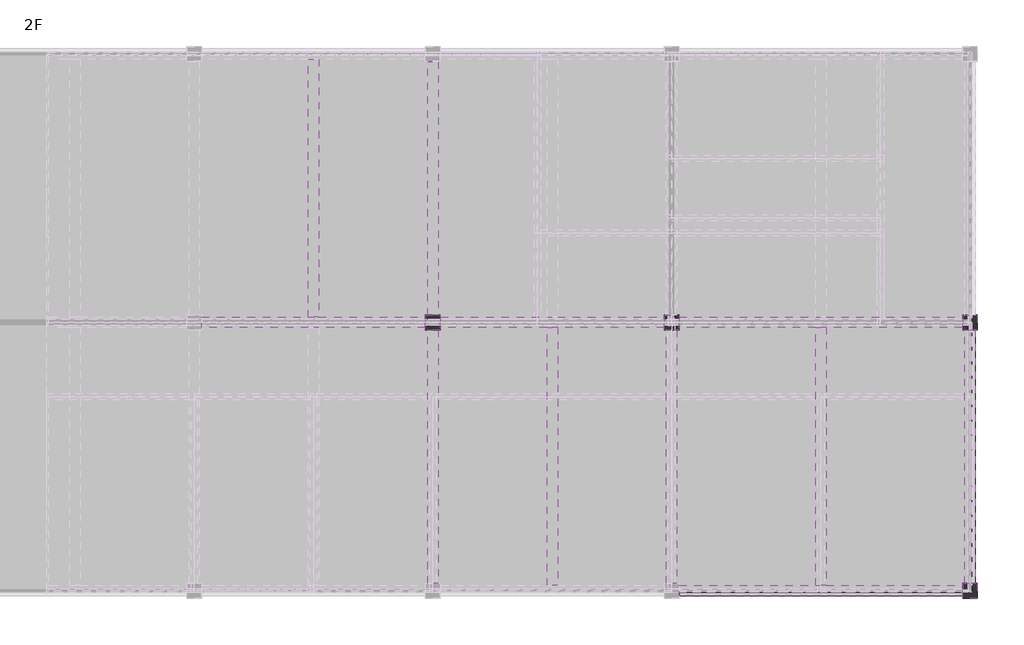
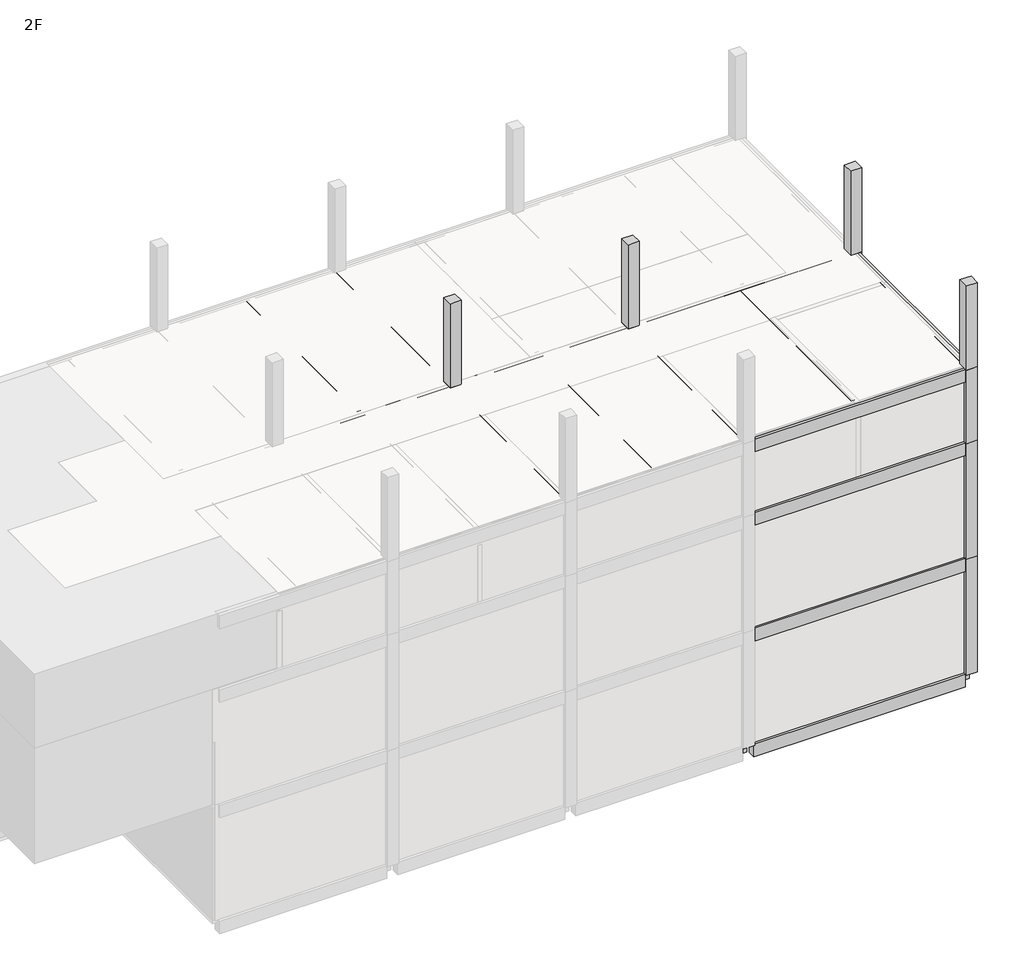
# One storey, part 6 of 7: 42 beams, 16 columns.
"""IFC4 building model written with IfcOpenShell, lengths in millimetres."""

from ifc_helpers import new_model, si_unit, frame, origin, place, context, project, spatial, polyline, outline, extrude, faceted_brep, element, save

model = new_model("IFC4")

# Units and contexts
model_context = context("Model", 3, world=origin())
ifc_project = project(units=[si_unit("LENGTHUNIT", "METRE", prefix="MILLI")], contexts=[model_context])

# Site, building, storey
site = spatial("IfcSite", under=ifc_project)
building = spatial("IfcBuilding", under=site)
storey = spatial("IfcBuildingStorey", under=building, Name="2F", Elevation=3500.0)

# Beams
placement = place(None, origin())
element("IfcBeam", 1, ObjectType="Concrete-Rectangular-Beam : BM111_400x500_RG1", at=placement, inside=storey, context=model_context, shape_type="SweptSolid", body=[
    extrude(outline(polyline([(65634.6521483, 173098.8614395), (65284.6521483, 173098.8614395), (65284.6521483, 181748.8614395), (65634.6521483, 181748.8614395), (65634.6521483, 173098.8614395)])), frame((0.0, 0.0, 2900.0), z_axis=(0.0, 0.0, 1.0), x_axis=(1.0, 0.0, 0.0)), (0.0, 0.0, 1.0), 600.0),
])
element("IfcBeam", 2, ObjectType="Concrete-Rectangular-Beam : BM111_400x500_RG1", at=placement, inside=storey, context=model_context, shape_type="SweptSolid", body=[
    extrude(outline(polyline([(73284.6521483, 172748.8614395), (73634.6521483, 172748.8614395), (73634.6521483, 164098.8614395), (73284.6521483, 164098.8614395), (73284.6521483, 172748.8614395)])), frame((0.0, 0.0, 2900.0), z_axis=(0.0, 0.0, 1.0), x_axis=(1.0, 0.0, 0.0)), (0.0, 0.0, 1.0), 600.0),
])
element("IfcBeam", 3, ObjectType="Concrete-Rectangular-Beam : BM111_400x500_RG1", at=placement, inside=storey, context=model_context, shape_type="SweptSolid", body=[
    extrude(outline(polyline([(82284.6521483, 172748.8614395), (82634.6521483, 172748.8614395), (82634.6521483, 164098.8614395), (82284.6521483, 164098.8614395), (82284.6521483, 172748.8614395)])), frame((0.0, 0.0, 2900.0), z_axis=(0.0, 0.0, 1.0), x_axis=(1.0, 0.0, 0.0)), (0.0, 0.0, 1.0), 600.0),
])
element("IfcBeam", 4, ObjectType="Concrete-Rectangular-Beam : BM111_400x500_RG1", at=placement, inside=storey, context=model_context, shape_type="SweptSolid", body=[
    extrude(outline(polyline([(65634.6521483, 173098.8614395), (65284.6521483, 173098.8614395), (65284.6521483, 181748.8614395), (65634.6521483, 181748.8614395), (65634.6521483, 173098.8614395)])), frame((0.0, 0.0, 8400.0), z_axis=(0.0, 0.0, 1.0), x_axis=(1.0, 0.0, 0.0)), (0.0, 0.0, 1.0), 600.0),
])
element("IfcBeam", 5, ObjectType="Concrete-Rectangular-Beam : BM111_400x500_RG1", at=placement, inside=storey, context=model_context, shape_type="SweptSolid", body=[
    extrude(outline(polyline([(73284.6521483, 172748.8614395), (73634.6521483, 172748.8614395), (73634.6521483, 164098.8614395), (73284.6521483, 164098.8614395), (73284.6521483, 172748.8614395)])), frame((0.0, 0.0, 8400.0), z_axis=(0.0, 0.0, 1.0), x_axis=(1.0, 0.0, 0.0)), (0.0, 0.0, 1.0), 600.0),
])
element("IfcBeam", 6, ObjectType="Concrete-Rectangular-Beam : BM111_400x500_RG1", at=placement, inside=storey, context=model_context, shape_type="SweptSolid", body=[
    extrude(outline(polyline([(82284.6521483, 172748.8614395), (82634.6521483, 172748.8614395), (82634.6521483, 164098.8614395), (82284.6521483, 164098.8614395), (82284.6521483, 172748.8614395)])), frame((0.0, 0.0, 8400.0), z_axis=(0.0, 0.0, 1.0), x_axis=(1.0, 0.0, 0.0)), (0.0, 0.0, 1.0), 600.0),
])
element("IfcBeam", 7, ObjectType="Concrete-Rectangular-Beam : BM111_400x500_RG1", at=placement, inside=storey, context=model_context, shape_type="SweptSolid", body=[
    extrude(outline(polyline([(65634.6521483, 173098.8614395), (65284.6521483, 173098.8614395), (65284.6521483, 181748.8614395), (65634.6521483, 181748.8614395), (65634.6521483, 173098.8614395)])), frame((0.0, 0.0, 13900.0), z_axis=(0.0, 0.0, 1.0), x_axis=(1.0, 0.0, 0.0)), (0.0, 0.0, 1.0), 600.0),
])
element("IfcBeam", 8, ObjectType="Concrete-Rectangular-Beam : BM111_400x500_RG1", at=placement, inside=storey, context=model_context, shape_type="SweptSolid", body=[
    extrude(outline(polyline([(73284.6521483, 172748.8614395), (73634.6521483, 172748.8614395), (73634.6521483, 164098.8614395), (73284.6521483, 164098.8614395), (73284.6521483, 172748.8614395)])), frame((0.0, 0.0, 13900.0), z_axis=(0.0, 0.0, 1.0), x_axis=(1.0, 0.0, 0.0)), (0.0, 0.0, 1.0), 600.0),
])
element("IfcBeam", 9, ObjectType="Concrete-Rectangular-Beam : BM111_400x500_RG1", at=placement, inside=storey, context=model_context, shape_type="SweptSolid", body=[
    extrude(outline(polyline([(82284.6521483, 172748.8614395), (82634.6521483, 172748.8614395), (82634.6521483, 164098.8614395), (82284.6521483, 164098.8614395), (82284.6521483, 172748.8614395)])), frame((0.0, 0.0, 13900.0), z_axis=(0.0, 0.0, 1.0), x_axis=(1.0, 0.0, 0.0)), (0.0, 0.0, 1.0), 600.0),
])
element("IfcBeam", 10, ObjectType="Concrete-Rectangular-Beam : BM111_400x500_RG1", at=placement, inside=storey, context=model_context, shape_type="SweptSolid", body=[
    extrude(outline(polyline([(65634.6521483, 173098.8614395), (65284.6521483, 173098.8614395), (65284.6521483, 181748.8614395), (65634.6521483, 181748.8614395), (65634.6521483, 173098.8614395)])), frame((0.0, 0.0, 17400.0), z_axis=(0.0, 0.0, 1.0), x_axis=(1.0, 0.0, 0.0)), (0.0, 0.0, 1.0), 600.0),
])
element("IfcBeam", 11, ObjectType="Concrete-Rectangular-Beam : BM111_400x500_RG1", at=placement, inside=storey, context=model_context, shape_type="SweptSolid", body=[
    extrude(outline(polyline([(73284.6521483, 172748.8614395), (73634.6521483, 172748.8614395), (73634.6521483, 164098.8614395), (73284.6521483, 164098.8614395), (73284.6521483, 172748.8614395)])), frame((0.0, 0.0, 17400.0), z_axis=(0.0, 0.0, 1.0), x_axis=(1.0, 0.0, 0.0)), (0.0, 0.0, 1.0), 600.0),
])
element("IfcBeam", 12, ObjectType="Concrete-Rectangular-Beam : BM111_400x500_RG1", at=placement, inside=storey, context=model_context, shape_type="SweptSolid", body=[
    extrude(outline(polyline([(82284.6521483, 172748.8614395), (82634.6521483, 172748.8614395), (82634.6521483, 164098.8614395), (82284.6521483, 164098.8614395), (82284.6521483, 172748.8614395)])), frame((0.0, 0.0, 17400.0), z_axis=(0.0, 0.0, 1.0), x_axis=(1.0, 0.0, 0.0)), (0.0, 0.0, 1.0), 600.0),
])
element("IfcBeam", 13, ObjectType="Concrete-Rectangular-Beam : BM111_400x500_RG1", at=placement, inside=storey, context=model_context, shape_type="Brep", body=[
    faceted_brep([(61709.6521483, 173098.8614395, 3500.0), (61709.6521483, 172748.8614395, 3500.0), (65284.6521483, 172748.8614395, 3500.0), (65634.6521483, 172748.8614395, 3500.0), (69209.6521483, 172748.8614395, 3500.0), (69209.6521483, 173098.8614395, 3500.0), (65634.6521483, 173098.8614395, 3500.0), (65284.6521483, 173098.8614395, 3500.0), (61709.6521483, 172748.8614395, 2900.0), (65284.6521483, 172748.8614395, 2900.0), (65634.6521483, 172748.8614395, 2900.0), (69209.6521483, 172748.8614395, 2900.0), (61709.6521483, 173098.8614395, 2900.0), (65284.6521483, 173098.8614395, 2900.0), (65634.6521483, 173098.8614395, 2900.0), (69209.6521483, 173098.8614395, 2900.0)], [[[0, 1, 2, 3, 4, 5, 6, 7]], [[1, 8, 9, 10, 11, 4, 3, 2]], [[8, 12, 13, 14, 15, 11, 10, 9]], [[12, 0, 7, 6, 5, 15, 14, 13]], [[1, 0, 12, 8]], [[5, 4, 11, 15]]]),
])
element("IfcBeam", 14, ObjectType="Concrete-Rectangular-Beam : BM111_400x500_RG1", at=placement, inside=storey, context=model_context, shape_type="Brep", body=[
    faceted_brep([(69709.6521483, 173098.8614395, 3500.0), (69709.6521483, 172748.8614395, 3500.0), (73284.6521483, 172748.8614395, 3500.0), (73634.6521483, 172748.8614395, 3500.0), (77209.6521483, 172748.8614395, 3500.0), (77209.6521483, 173098.8614395, 3500.0), (73634.6521483, 173098.8614395, 3500.0), (73284.6521483, 173098.8614395, 3500.0), (69709.6521483, 172748.8614395, 2900.0), (73284.6521483, 172748.8614395, 2900.0), (73634.6521483, 172748.8614395, 2900.0), (77209.6521483, 172748.8614395, 2900.0), (69709.6521483, 173098.8614395, 2900.0), (73284.6521483, 173098.8614395, 2900.0), (73634.6521483, 173098.8614395, 2900.0), (77209.6521483, 173098.8614395, 2900.0)], [[[0, 1, 2, 3, 4, 5, 6, 7]], [[1, 8, 9, 10, 11, 4, 3, 2]], [[8, 12, 13, 14, 15, 11, 10, 9]], [[12, 0, 7, 6, 5, 15, 14, 13]], [[1, 0, 12, 8]], [[5, 4, 11, 15]]]),
])
element("IfcBeam", 15, ObjectType="Concrete-Rectangular-Beam : BM111_400x500_RG1", at=placement, inside=storey, context=model_context, shape_type="Brep", body=[
    faceted_brep([(77709.6521483, 173098.8614395, 3500.0), (77709.6521483, 172748.8614395, 3500.0), (82284.6521483, 172748.8614395, 3500.0), (82634.6521483, 172748.8614395, 3500.0), (87209.6521483, 172748.8614395, 3500.0), (87209.6521483, 173098.8614395, 3500.0), (82634.6521483, 173098.8614395, 3500.0), (82284.6521483, 173098.8614395, 3500.0), (77709.6521483, 172748.8614395, 2900.0), (82284.6521483, 172748.8614395, 2900.0), (82634.6521483, 172748.8614395, 2900.0), (87209.6521483, 172748.8614395, 2900.0), (77709.6521483, 173098.8614395, 2900.0), (82284.6521483, 173098.8614395, 2900.0), (82634.6521483, 173098.8614395, 2900.0), (87209.6521483, 173098.8614395, 2900.0)], [[[0, 1, 2, 3, 4, 5, 6, 7]], [[1, 8, 9, 10, 11, 4, 3, 2]], [[8, 12, 13, 14, 15, 11, 10, 9]], [[12, 0, 7, 6, 5, 15, 14, 13]], [[1, 0, 12, 8]], [[5, 4, 11, 15]]]),
])
element("IfcBeam", 16, ObjectType="Concrete-Rectangular-Beam : BM111_400x500_RG1", at=placement, inside=storey, context=model_context, shape_type="Brep", body=[
    faceted_brep([(77709.6521483, 164098.8614395, 3500.0), (77709.6521483, 163748.8614395, 3500.0), (87209.6521483, 163748.8614395, 3500.0), (87209.6521483, 164098.8614395, 3500.0), (82634.6521483, 164098.8614395, 3500.0), (82284.6521483, 164098.8614395, 3500.0), (77709.6521483, 163748.8614395, 2900.0), (87209.6521483, 163748.8614395, 2900.0), (77709.6521483, 164098.8614395, 2900.0), (82284.6521483, 164098.8614395, 2900.0), (82634.6521483, 164098.8614395, 2900.0), (87209.6521483, 164098.8614395, 2900.0)], [[[0, 1, 2, 3, 4, 5]], [[1, 6, 7, 2]], [[6, 8, 9, 10, 11, 7]], [[8, 0, 5, 4, 3, 11, 10, 9]], [[1, 0, 8, 6]], [[3, 2, 7, 11]]]),
])
element("IfcBeam", 17, ObjectType="Concrete-Rectangular-Beam : BM111_400x500_RG1", at=placement, inside=storey, context=model_context, shape_type="Brep", body=[
    faceted_brep([(61709.6521483, 173098.8614395, 9000.0), (61709.6521483, 172748.8614395, 9000.0), (65284.6521483, 172748.8614395, 9000.0), (65634.6521483, 172748.8614395, 9000.0), (69209.6521483, 172748.8614395, 9000.0), (69209.6521483, 173098.8614395, 9000.0), (65634.6521483, 173098.8614395, 9000.0), (65284.6521483, 173098.8614395, 9000.0), (61709.6521483, 172748.8614395, 8400.0), (65284.6521483, 172748.8614395, 8400.0), (65634.6521483, 172748.8614395, 8400.0), (69209.6521483, 172748.8614395, 8400.0), (61709.6521483, 173098.8614395, 8400.0), (65284.6521483, 173098.8614395, 8400.0), (65634.6521483, 173098.8614395, 8400.0), (69209.6521483, 173098.8614395, 8400.0)], [[[0, 1, 2, 3, 4, 5, 6, 7]], [[1, 8, 9, 10, 11, 4, 3, 2]], [[8, 12, 13, 14, 15, 11, 10, 9]], [[12, 0, 7, 6, 5, 15, 14, 13]], [[1, 0, 12, 8]], [[5, 4, 11, 15]]]),
])
element("IfcBeam", 18, ObjectType="Concrete-Rectangular-Beam : BM111_400x500_RG1", at=placement, inside=storey, context=model_context, shape_type="Brep", body=[
    faceted_brep([(69709.6521483, 173098.8614395, 9000.0), (69709.6521483, 172748.8614395, 9000.0), (73284.6521483, 172748.8614395, 9000.0), (73634.6521483, 172748.8614395, 9000.0), (77209.6521483, 172748.8614395, 9000.0), (77209.6521483, 173098.8614395, 9000.0), (73634.6521483, 173098.8614395, 9000.0), (73284.6521483, 173098.8614395, 9000.0), (69709.6521483, 172748.8614395, 8400.0), (73284.6521483, 172748.8614395, 8400.0), (73634.6521483, 172748.8614395, 8400.0), (77209.6521483, 172748.8614395, 8400.0), (69709.6521483, 173098.8614395, 8400.0), (73284.6521483, 173098.8614395, 8400.0), (73634.6521483, 173098.8614395, 8400.0), (77209.6521483, 173098.8614395, 8400.0)], [[[0, 1, 2, 3, 4, 5, 6, 7]], [[1, 8, 9, 10, 11, 4, 3, 2]], [[8, 12, 13, 14, 15, 11, 10, 9]], [[12, 0, 7, 6, 5, 15, 14, 13]], [[1, 0, 12, 8]], [[5, 4, 11, 15]]]),
])
element("IfcBeam", 19, ObjectType="Concrete-Rectangular-Beam : BM111_400x500_RG1", at=placement, inside=storey, context=model_context, shape_type="Brep", body=[
    faceted_brep([(77709.6521483, 173098.8614395, 9000.0), (77709.6521483, 172748.8614395, 9000.0), (82284.6521483, 172748.8614395, 9000.0), (82634.6521483, 172748.8614395, 9000.0), (87209.6521483, 172748.8614395, 9000.0), (87209.6521483, 173098.8614395, 9000.0), (82634.6521483, 173098.8614395, 9000.0), (82284.6521483, 173098.8614395, 9000.0), (77709.6521483, 172748.8614395, 8400.0), (82284.6521483, 172748.8614395, 8400.0), (82634.6521483, 172748.8614395, 8400.0), (87209.6521483, 172748.8614395, 8400.0), (77709.6521483, 173098.8614395, 8400.0), (82284.6521483, 173098.8614395, 8400.0), (82634.6521483, 173098.8614395, 8400.0), (87209.6521483, 173098.8614395, 8400.0)], [[[0, 1, 2, 3, 4, 5, 6, 7]], [[1, 8, 9, 10, 11, 4, 3, 2]], [[8, 12, 13, 14, 15, 11, 10, 9]], [[12, 0, 7, 6, 5, 15, 14, 13]], [[1, 0, 12, 8]], [[5, 4, 11, 15]]]),
])
element("IfcBeam", 20, ObjectType="Concrete-Rectangular-Beam : BM111_400x500_RG1", at=placement, inside=storey, context=model_context, shape_type="Brep", body=[
    faceted_brep([(77709.6521483, 164098.8614395, 9000.0), (77709.6521483, 163748.8614395, 9000.0), (87209.6521483, 163748.8614395, 9000.0), (87209.6521483, 164098.8614395, 9000.0), (82634.6521483, 164098.8614395, 9000.0), (82284.6521483, 164098.8614395, 9000.0), (77709.6521483, 163748.8614395, 8400.0), (87209.6521483, 163748.8614395, 8400.0), (77709.6521483, 164098.8614395, 8400.0), (82284.6521483, 164098.8614395, 8400.0), (82634.6521483, 164098.8614395, 8400.0), (87209.6521483, 164098.8614395, 8400.0)], [[[0, 1, 2, 3, 4, 5]], [[1, 6, 7, 2]], [[6, 8, 9, 10, 11, 7]], [[8, 0, 5, 4, 3, 11, 10, 9]], [[1, 0, 8, 6]], [[3, 2, 7, 11]]]),
])
element("IfcBeam", 21, ObjectType="Concrete-Rectangular-Beam : BM111_400x500_RG1", at=placement, inside=storey, context=model_context, shape_type="Brep", body=[
    faceted_brep([(61709.6521483, 173098.8614395, 14500.0), (61709.6521483, 172748.8614395, 14500.0), (65284.6521483, 172748.8614395, 14500.0), (65634.6521483, 172748.8614395, 14500.0), (69209.6521483, 172748.8614395, 14500.0), (69209.6521483, 173098.8614395, 14500.0), (65634.6521483, 173098.8614395, 14500.0), (65284.6521483, 173098.8614395, 14500.0), (61709.6521483, 172748.8614395, 13900.0), (65284.6521483, 172748.8614395, 13900.0), (65634.6521483, 172748.8614395, 13900.0), (69209.6521483, 172748.8614395, 13900.0), (61709.6521483, 173098.8614395, 13900.0), (65284.6521483, 173098.8614395, 13900.0), (65634.6521483, 173098.8614395, 13900.0), (69209.6521483, 173098.8614395, 13900.0)], [[[0, 1, 2, 3, 4, 5, 6, 7]], [[1, 8, 9, 10, 11, 4, 3, 2]], [[8, 12, 13, 14, 15, 11, 10, 9]], [[12, 0, 7, 6, 5, 15, 14, 13]], [[1, 0, 12, 8]], [[5, 4, 11, 15]]]),
])
element("IfcBeam", 22, ObjectType="Concrete-Rectangular-Beam : BM111_400x500_RG1", at=placement, inside=storey, context=model_context, shape_type="Brep", body=[
    faceted_brep([(69709.6521483, 173098.8614395, 14500.0), (69709.6521483, 172748.8614395, 14500.0), (73284.6521483, 172748.8614395, 14500.0), (73634.6521483, 172748.8614395, 14500.0), (77209.6521483, 172748.8614395, 14500.0), (77209.6521483, 173098.8614395, 14500.0), (73634.6521483, 173098.8614395, 14500.0), (73284.6521483, 173098.8614395, 14500.0), (69709.6521483, 172748.8614395, 13900.0), (73284.6521483, 172748.8614395, 13900.0), (73634.6521483, 172748.8614395, 13900.0), (77209.6521483, 172748.8614395, 13900.0), (69709.6521483, 173098.8614395, 13900.0), (73284.6521483, 173098.8614395, 13900.0), (73634.6521483, 173098.8614395, 13900.0), (77209.6521483, 173098.8614395, 13900.0)], [[[0, 1, 2, 3, 4, 5, 6, 7]], [[1, 8, 9, 10, 11, 4, 3, 2]], [[8, 12, 13, 14, 15, 11, 10, 9]], [[12, 0, 7, 6, 5, 15, 14, 13]], [[1, 0, 12, 8]], [[5, 4, 11, 15]]]),
])
element("IfcBeam", 23, ObjectType="Concrete-Rectangular-Beam : BM111_400x500_RG1", at=placement, inside=storey, context=model_context, shape_type="Brep", body=[
    faceted_brep([(77709.6521483, 173098.8614395, 14500.0), (77709.6521483, 172748.8614395, 14500.0), (82284.6521483, 172748.8614395, 14500.0), (82634.6521483, 172748.8614395, 14500.0), (87209.6521483, 172748.8614395, 14500.0), (87209.6521483, 173098.8614395, 14500.0), (82634.6521483, 173098.8614395, 14500.0), (82284.6521483, 173098.8614395, 14500.0), (77709.6521483, 172748.8614395, 13900.0), (82284.6521483, 172748.8614395, 13900.0), (82634.6521483, 172748.8614395, 13900.0), (87209.6521483, 172748.8614395, 13900.0), (77709.6521483, 173098.8614395, 13900.0), (82284.6521483, 173098.8614395, 13900.0), (82634.6521483, 173098.8614395, 13900.0), (87209.6521483, 173098.8614395, 13900.0)], [[[0, 1, 2, 3, 4, 5, 6, 7]], [[1, 8, 9, 10, 11, 4, 3, 2]], [[8, 12, 13, 14, 15, 11, 10, 9]], [[12, 0, 7, 6, 5, 15, 14, 13]], [[1, 0, 12, 8]], [[5, 4, 11, 15]]]),
])
element("IfcBeam", 24, ObjectType="Concrete-Rectangular-Beam : BM111_400x500_RG1", at=placement, inside=storey, context=model_context, shape_type="Brep", body=[
    faceted_brep([(77709.6521483, 164098.8614395, 14500.0), (77709.6521483, 163748.8614395, 14500.0), (87209.6521483, 163748.8614395, 14500.0), (87209.6521483, 164098.8614395, 14500.0), (82634.6521483, 164098.8614395, 14500.0), (82284.6521483, 164098.8614395, 14500.0), (77709.6521483, 163748.8614395, 13900.0), (87209.6521483, 163748.8614395, 13900.0), (77709.6521483, 164098.8614395, 13900.0), (82284.6521483, 164098.8614395, 13900.0), (82634.6521483, 164098.8614395, 13900.0), (87209.6521483, 164098.8614395, 13900.0)], [[[0, 1, 2, 3, 4, 5]], [[1, 6, 7, 2]], [[6, 8, 9, 10, 11, 7]], [[8, 0, 5, 4, 3, 11, 10, 9]], [[1, 0, 8, 6]], [[3, 2, 7, 11]]]),
])
element("IfcBeam", 25, ObjectType="Concrete-Rectangular-Beam : BM111_400x500_RG1", at=placement, inside=storey, context=model_context, shape_type="Brep", body=[
    faceted_brep([(61709.6521483, 173098.8614395, 18000.0), (61709.6521483, 172748.8614395, 18000.0), (65284.6521483, 172748.8614395, 18000.0), (65634.6521483, 172748.8614395, 18000.0), (69209.6521483, 172748.8614395, 18000.0), (69209.6521483, 173098.8614395, 18000.0), (65634.6521483, 173098.8614395, 18000.0), (65284.6521483, 173098.8614395, 18000.0), (61709.6521483, 172748.8614395, 17400.0), (65284.6521483, 172748.8614395, 17400.0), (65634.6521483, 172748.8614395, 17400.0), (69209.6521483, 172748.8614395, 17400.0), (61709.6521483, 173098.8614395, 17400.0), (65284.6521483, 173098.8614395, 17400.0), (65634.6521483, 173098.8614395, 17400.0), (69209.6521483, 173098.8614395, 17400.0)], [[[0, 1, 2, 3, 4, 5, 6, 7]], [[1, 8, 9, 10, 11, 4, 3, 2]], [[8, 12, 13, 14, 15, 11, 10, 9]], [[12, 0, 7, 6, 5, 15, 14, 13]], [[1, 0, 12, 8]], [[5, 4, 11, 15]]]),
])
element("IfcBeam", 26, ObjectType="Concrete-Rectangular-Beam : BM111_400x500_RG1", at=placement, inside=storey, context=model_context, shape_type="Brep", body=[
    faceted_brep([(69709.6521483, 173098.8614395, 18000.0), (69709.6521483, 172748.8614395, 18000.0), (73284.6521483, 172748.8614395, 18000.0), (73634.6521483, 172748.8614395, 18000.0), (77209.6521483, 172748.8614395, 18000.0), (77209.6521483, 173098.8614395, 18000.0), (73634.6521483, 173098.8614395, 18000.0), (73284.6521483, 173098.8614395, 18000.0), (69709.6521483, 172748.8614395, 17400.0), (73284.6521483, 172748.8614395, 17400.0), (73634.6521483, 172748.8614395, 17400.0), (77209.6521483, 172748.8614395, 17400.0), (69709.6521483, 173098.8614395, 17400.0), (73284.6521483, 173098.8614395, 17400.0), (73634.6521483, 173098.8614395, 17400.0), (77209.6521483, 173098.8614395, 17400.0)], [[[0, 1, 2, 3, 4, 5, 6, 7]], [[1, 8, 9, 10, 11, 4, 3, 2]], [[8, 12, 13, 14, 15, 11, 10, 9]], [[12, 0, 7, 6, 5, 15, 14, 13]], [[1, 0, 12, 8]], [[5, 4, 11, 15]]]),
])
element("IfcBeam", 27, ObjectType="Concrete-Rectangular-Beam : BM111_400x500_RG1", at=placement, inside=storey, context=model_context, shape_type="Brep", body=[
    faceted_brep([(77709.6521483, 173098.8614395, 18000.0), (77709.6521483, 172748.8614395, 18000.0), (82284.6521483, 172748.8614395, 18000.0), (82634.6521483, 172748.8614395, 18000.0), (87209.6521483, 172748.8614395, 18000.0), (87209.6521483, 173098.8614395, 18000.0), (82634.6521483, 173098.8614395, 18000.0), (82284.6521483, 173098.8614395, 18000.0), (77709.6521483, 172748.8614395, 17400.0), (82284.6521483, 172748.8614395, 17400.0), (82634.6521483, 172748.8614395, 17400.0), (87209.6521483, 172748.8614395, 17400.0), (77709.6521483, 173098.8614395, 17400.0), (82284.6521483, 173098.8614395, 17400.0), (82634.6521483, 173098.8614395, 17400.0), (87209.6521483, 173098.8614395, 17400.0)], [[[0, 1, 2, 3, 4, 5, 6, 7]], [[1, 8, 9, 10, 11, 4, 3, 2]], [[8, 12, 13, 14, 15, 11, 10, 9]], [[12, 0, 7, 6, 5, 15, 14, 13]], [[1, 0, 12, 8]], [[5, 4, 11, 15]]]),
])
element("IfcBeam", 28, ObjectType="Concrete-Rectangular-Beam : BM111_400x500_RG1", at=placement, inside=storey, context=model_context, shape_type="Brep", body=[
    faceted_brep([(77709.6521483, 164098.8614395, 18000.0), (77709.6521483, 163748.8614395, 18000.0), (87209.6521483, 163748.8614395, 18000.0), (87209.6521483, 164098.8614395, 18000.0), (82634.6521483, 164098.8614395, 18000.0), (82284.6521483, 164098.8614395, 18000.0), (77709.6521483, 163748.8614395, 17400.0), (87209.6521483, 163748.8614395, 17400.0), (77709.6521483, 164098.8614395, 17400.0), (82284.6521483, 164098.8614395, 17400.0), (82634.6521483, 164098.8614395, 17400.0), (87209.6521483, 164098.8614395, 17400.0)], [[[0, 1, 2, 3, 4, 5]], [[1, 6, 7, 2]], [[6, 8, 9, 10, 11, 7]], [[8, 0, 5, 4, 3, 11, 10, 9]], [[1, 0, 8, 6]], [[3, 2, 7, 11]]]),
])
element("IfcBeam", 29, ObjectType="Concrete-Rectangular-Beam : BM111_400x500_RG1", at=placement, inside=storey, context=model_context, shape_type="SweptSolid", body=[
    extrude(outline(polyline([(69284.6521483, 181673.8614395), (69634.6521483, 181673.8614395), (69634.6521483, 173173.8614395), (69284.6521483, 173173.8614395), (69284.6521483, 181673.8614395)])), frame((0.0, 0.0, 2900.0), z_axis=(0.0, 0.0, 1.0), x_axis=(1.0, 0.0, 0.0)), (0.0, 0.0, 1.0), 600.0),
])
element("IfcBeam", 30, ObjectType="Concrete-Rectangular-Beam : BM111_400x500_RG1", at=placement, inside=storey, context=model_context, shape_type="SweptSolid", body=[
    extrude(outline(polyline([(77284.6521483, 172673.8614395), (77634.6521483, 172673.8614395), (77634.6521483, 164173.8614395), (77284.6521483, 164173.8614395), (77284.6521483, 172673.8614395)])), frame((0.0, 0.0, 2900.0), z_axis=(0.0, 0.0, 1.0), x_axis=(1.0, 0.0, 0.0)), (0.0, 0.0, 1.0), 600.0),
])
element("IfcBeam", 31, ObjectType="Concrete-Rectangular-Beam : BM111_400x500_RG1", at=placement, inside=storey, context=model_context, shape_type="SweptSolid", body=[
    extrude(outline(polyline([(87284.6521483, 172673.8614395), (87634.6521483, 172673.8614395), (87634.6521483, 164173.8614395), (87284.6521483, 164173.8614395), (87284.6521483, 172673.8614395)])), frame((0.0, 0.0, 2900.0), z_axis=(0.0, 0.0, 1.0), x_axis=(1.0, 0.0, 0.0)), (0.0, 0.0, 1.0), 600.0),
])
element("IfcBeam", 32, ObjectType="Concrete-Rectangular-Beam : BM111_400x500_RG1", at=placement, inside=storey, context=model_context, shape_type="SweptSolid", body=[
    extrude(outline(polyline([(69284.6521483, 181673.8614395), (69634.6521483, 181673.8614395), (69634.6521483, 173173.8614395), (69284.6521483, 173173.8614395), (69284.6521483, 181673.8614395)])), frame((0.0, 0.0, 8400.0), z_axis=(0.0, 0.0, 1.0), x_axis=(1.0, 0.0, 0.0)), (0.0, 0.0, 1.0), 600.0),
])
element("IfcBeam", 33, ObjectType="Concrete-Rectangular-Beam : BM111_400x500_RG1", at=placement, inside=storey, context=model_context, shape_type="SweptSolid", body=[
    extrude(outline(polyline([(77284.6521483, 172673.8614395), (77634.6521483, 172673.8614395), (77634.6521483, 164173.8614395), (77284.6521483, 164173.8614395), (77284.6521483, 172673.8614395)])), frame((0.0, 0.0, 8400.0), z_axis=(0.0, 0.0, 1.0), x_axis=(1.0, 0.0, 0.0)), (0.0, 0.0, 1.0), 600.0),
])
element("IfcBeam", 34, ObjectType="Concrete-Rectangular-Beam : BM111_400x500_RG1", at=placement, inside=storey, context=model_context, shape_type="SweptSolid", body=[
    extrude(outline(polyline([(87284.6521483, 172673.8614395), (87634.6521483, 172673.8614395), (87634.6521483, 164173.8614395), (87284.6521483, 164173.8614395), (87284.6521483, 172673.8614395)])), frame((0.0, 0.0, 8400.0), z_axis=(0.0, 0.0, 1.0), x_axis=(1.0, 0.0, 0.0)), (0.0, 0.0, 1.0), 600.0),
])
element("IfcBeam", 35, ObjectType="Concrete-Rectangular-Beam : BM111_400x500_RG1", at=placement, inside=storey, context=model_context, shape_type="SweptSolid", body=[
    extrude(outline(polyline([(69284.6521483, 181673.8614395), (69634.6521483, 181673.8614395), (69634.6521483, 173173.8614395), (69284.6521483, 173173.8614395), (69284.6521483, 181673.8614395)])), frame((0.0, 0.0, 13900.0), z_axis=(0.0, 0.0, 1.0), x_axis=(1.0, 0.0, 0.0)), (0.0, 0.0, 1.0), 600.0),
])
element("IfcBeam", 36, ObjectType="Concrete-Rectangular-Beam : BM111_400x500_RG1", at=placement, inside=storey, context=model_context, shape_type="SweptSolid", body=[
    extrude(outline(polyline([(69284.6521483, 172673.8614395), (69634.6521483, 172673.8614395), (69634.6521483, 164173.8614395), (69284.6521483, 164173.8614395), (69284.6521483, 172673.8614395)])), frame((0.0, 0.0, 13900.0), z_axis=(0.0, 0.0, 1.0), x_axis=(1.0, 0.0, 0.0)), (0.0, 0.0, 1.0), 600.0),
])
element("IfcBeam", 37, ObjectType="Concrete-Rectangular-Beam : BM111_400x500_RG1", at=placement, inside=storey, context=model_context, shape_type="SweptSolid", body=[
    extrude(outline(polyline([(77284.6521483, 172673.8614395), (77634.6521483, 172673.8614395), (77634.6521483, 164173.8614395), (77284.6521483, 164173.8614395), (77284.6521483, 172673.8614395)])), frame((0.0, 0.0, 13900.0), z_axis=(0.0, 0.0, 1.0), x_axis=(1.0, 0.0, 0.0)), (0.0, 0.0, 1.0), 600.0),
])
element("IfcBeam", 38, ObjectType="Concrete-Rectangular-Beam : BM111_400x500_RG1", at=placement, inside=storey, context=model_context, shape_type="SweptSolid", body=[
    extrude(outline(polyline([(87284.6521483, 172673.8614395), (87634.6521483, 172673.8614395), (87634.6521483, 164173.8614395), (87284.6521483, 164173.8614395), (87284.6521483, 172673.8614395)])), frame((0.0, 0.0, 13900.0), z_axis=(0.0, 0.0, 1.0), x_axis=(1.0, 0.0, 0.0)), (0.0, 0.0, 1.0), 600.0),
])
element("IfcBeam", 39, ObjectType="Concrete-Rectangular-Beam : BM111_400x500_RG1", at=placement, inside=storey, context=model_context, shape_type="SweptSolid", body=[
    extrude(outline(polyline([(69284.6521483, 181673.8614395), (69634.6521483, 181673.8614395), (69634.6521483, 173173.8614395), (69284.6521483, 173173.8614395), (69284.6521483, 181673.8614395)])), frame((0.0, 0.0, 17400.0), z_axis=(0.0, 0.0, 1.0), x_axis=(1.0, 0.0, 0.0)), (0.0, 0.0, 1.0), 600.0),
])
element("IfcBeam", 40, ObjectType="Concrete-Rectangular-Beam : BM111_400x500_RG1", at=placement, inside=storey, context=model_context, shape_type="SweptSolid", body=[
    extrude(outline(polyline([(69284.6521483, 172673.8614395), (69634.6521483, 172673.8614395), (69634.6521483, 164173.8614395), (69284.6521483, 164173.8614395), (69284.6521483, 172673.8614395)])), frame((0.0, 0.0, 17400.0), z_axis=(0.0, 0.0, 1.0), x_axis=(1.0, 0.0, 0.0)), (0.0, 0.0, 1.0), 600.0),
])
element("IfcBeam", 41, ObjectType="Concrete-Rectangular-Beam : BM111_400x500_RG1", at=placement, inside=storey, context=model_context, shape_type="SweptSolid", body=[
    extrude(outline(polyline([(77284.6521483, 172673.8614395), (77634.6521483, 172673.8614395), (77634.6521483, 164173.8614395), (77284.6521483, 164173.8614395), (77284.6521483, 172673.8614395)])), frame((0.0, 0.0, 17400.0), z_axis=(0.0, 0.0, 1.0), x_axis=(1.0, 0.0, 0.0)), (0.0, 0.0, 1.0), 600.0),
])
element("IfcBeam", 42, ObjectType="Concrete-Rectangular-Beam : BM111_400x500_RG1", at=placement, inside=storey, context=model_context, shape_type="SweptSolid", body=[
    extrude(outline(polyline([(87284.6521483, 172673.8614395), (87634.6521483, 172673.8614395), (87634.6521483, 164173.8614395), (87284.6521483, 164173.8614395), (87284.6521483, 172673.8614395)])), frame((0.0, 0.0, 17400.0), z_axis=(0.0, 0.0, 1.0), x_axis=(1.0, 0.0, 0.0)), (0.0, 0.0, 1.0), 600.0),
])

# Columns
element("IfcColumn", 43, ObjectType="Concrete-Rectangular-Column : CL111_500x500", at=placement, inside=storey, context=model_context, shape_type="Brep", body=[
    faceted_brep([(69709.6521483, 173173.8614395, 3500.0), (69709.6521483, 172673.8614395, 3500.0), (69209.6521483, 172673.8614395, 3500.0), (69209.6521483, 173173.8614395, 3500.0), (69709.6521483, 173173.8614395, 9000.0), (69709.6521483, 173098.8614395, 9000.0), (69709.6521483, 172748.8614395, 9000.0), (69709.6521483, 172673.8614395, 9000.0), (69634.6521483, 172673.8614395, 9000.0), (69284.6521483, 172673.8614395, 9000.0), (69209.6521483, 172673.8614395, 9000.0), (69209.6521483, 172748.8614395, 9000.0), (69209.6521483, 173098.8614395, 9000.0), (69209.6521483, 173173.8614395, 9000.0), (69284.6521483, 173173.8614395, 9000.0), (69634.6521483, 173173.8614395, 9000.0)], [[[0, 1, 2, 3]], [[4, 5, 6, 7, 1, 0]], [[7, 8, 9, 10, 2, 1]], [[10, 11, 12, 13, 3, 2]], [[13, 14, 15, 4, 0, 3]], [[4, 15, 14, 13, 12, 11, 10, 9, 8, 7, 6, 5]]]),
])
element("IfcColumn", 44, ObjectType="Concrete-Rectangular-Column : CL111_500x500", at=placement, inside=storey, context=model_context, shape_type="Brep", body=[
    faceted_brep([(69709.6521483, 173173.8614395, 9000.0), (69709.6521483, 172673.8614395, 9000.0), (69209.6521483, 172673.8614395, 9000.0), (69209.6521483, 173173.8614395, 9000.0), (69709.6521483, 173173.8614395, 14500.0), (69709.6521483, 173098.8614395, 14500.0), (69709.6521483, 172748.8614395, 14500.0), (69709.6521483, 172673.8614395, 14500.0), (69634.6521483, 172673.8614395, 14500.0), (69284.6521483, 172673.8614395, 14500.0), (69209.6521483, 172673.8614395, 14500.0), (69209.6521483, 172748.8614395, 14500.0), (69209.6521483, 173098.8614395, 14500.0), (69209.6521483, 173173.8614395, 14500.0), (69284.6521483, 173173.8614395, 14500.0), (69634.6521483, 173173.8614395, 14500.0)], [[[0, 1, 2, 3]], [[4, 5, 6, 7, 1, 0]], [[7, 8, 9, 10, 2, 1]], [[10, 11, 12, 13, 3, 2]], [[13, 14, 15, 4, 0, 3]], [[4, 15, 14, 13, 12, 11, 10, 9, 8, 7, 6, 5]]]),
])
element("IfcColumn", 45, ObjectType="Concrete-Rectangular-Column : CL111_500x500", at=placement, inside=storey, context=model_context, shape_type="Brep", body=[
    faceted_brep([(69709.6521483, 173173.8614395, 14500.0), (69709.6521483, 172673.8614395, 14500.0), (69209.6521483, 172673.8614395, 14500.0), (69209.6521483, 173173.8614395, 14500.0), (69709.6521483, 173173.8614395, 18000.0), (69709.6521483, 173098.8614395, 18000.0), (69709.6521483, 172748.8614395, 18000.0), (69709.6521483, 172673.8614395, 18000.0), (69634.6521483, 172673.8614395, 18000.0), (69284.6521483, 172673.8614395, 18000.0), (69209.6521483, 172673.8614395, 18000.0), (69209.6521483, 172748.8614395, 18000.0), (69209.6521483, 173098.8614395, 18000.0), (69209.6521483, 173173.8614395, 18000.0), (69284.6521483, 173173.8614395, 18000.0), (69634.6521483, 173173.8614395, 18000.0)], [[[0, 1, 2, 3]], [[4, 5, 6, 7, 1, 0]], [[7, 8, 9, 10, 2, 1]], [[10, 11, 12, 13, 3, 2]], [[13, 14, 15, 4, 0, 3]], [[4, 15, 14, 13, 12, 11, 10, 9, 8, 7, 6, 5]]]),
])
element("IfcColumn", 46, ObjectType="Concrete-Rectangular-Column : CL111_500x500", at=placement, inside=storey, context=model_context, shape_type="SweptSolid", body=[
    extrude(outline(polyline([(69709.6521483, 173173.8614395), (69709.6521483, 172673.8614395), (69209.6521483, 172673.8614395), (69209.6521483, 173173.8614395), (69709.6521483, 173173.8614395)])), frame((0.0, 0.0, 18000.0), z_axis=(0.0, 0.0, 1.0), x_axis=(1.0, 0.0, 0.0)), (0.0, 0.0, 1.0), 4000.0),
])
element("IfcColumn", 47, ObjectType="Concrete-Rectangular-Column : CL111_500x500", at=placement, inside=storey, context=model_context, shape_type="Brep", body=[
    faceted_brep([(77709.6521483, 173173.8614395, 3500.0), (77709.6521483, 172673.8614395, 3500.0), (77209.6521483, 172673.8614395, 3500.0), (77209.6521483, 173173.8614395, 3500.0), (77709.6521483, 173173.8614395, 9000.0), (77709.6521483, 173098.8614395, 9000.0), (77709.6521483, 172748.8614395, 9000.0), (77709.6521483, 172673.8614395, 9000.0), (77634.6521483, 172673.8614395, 9000.0), (77284.6521483, 172673.8614395, 9000.0), (77209.6521483, 172673.8614395, 9000.0), (77209.6521483, 172748.8614395, 9000.0), (77209.6521483, 173098.8614395, 9000.0), (77209.6521483, 173173.8614395, 9000.0), (77284.6521483, 173173.8614395, 9000.0), (77634.6521483, 173173.8614395, 9000.0)], [[[0, 1, 2, 3]], [[4, 5, 6, 7, 1, 0]], [[7, 8, 9, 10, 2, 1]], [[10, 11, 12, 13, 3, 2]], [[13, 14, 15, 4, 0, 3]], [[4, 15, 14, 13, 12, 11, 10, 9, 8, 7, 6, 5]]]),
])
element("IfcColumn", 48, ObjectType="Concrete-Rectangular-Column : CL111_500x500", at=placement, inside=storey, context=model_context, shape_type="Brep", body=[
    faceted_brep([(77709.6521483, 173173.8614395, 9000.0), (77709.6521483, 172673.8614395, 9000.0), (77209.6521483, 172673.8614395, 9000.0), (77209.6521483, 173173.8614395, 9000.0), (77709.6521483, 173173.8614395, 14500.0), (77709.6521483, 173098.8614395, 14500.0), (77709.6521483, 172748.8614395, 14500.0), (77709.6521483, 172673.8614395, 14500.0), (77634.6521483, 172673.8614395, 14500.0), (77284.6521483, 172673.8614395, 14500.0), (77209.6521483, 172673.8614395, 14500.0), (77209.6521483, 172748.8614395, 14500.0), (77209.6521483, 173098.8614395, 14500.0), (77209.6521483, 173173.8614395, 14500.0), (77284.6521483, 173173.8614395, 14500.0), (77634.6521483, 173173.8614395, 14500.0)], [[[0, 1, 2, 3]], [[4, 5, 6, 7, 1, 0]], [[7, 8, 9, 10, 2, 1]], [[10, 11, 12, 13, 3, 2]], [[13, 14, 15, 4, 0, 3]], [[4, 15, 14, 13, 12, 11, 10, 9, 8, 7, 6, 5]]]),
])
element("IfcColumn", 49, ObjectType="Concrete-Rectangular-Column : CL111_500x500", at=placement, inside=storey, context=model_context, shape_type="Brep", body=[
    faceted_brep([(77709.6521483, 173173.8614395, 14500.0), (77709.6521483, 172673.8614395, 14500.0), (77209.6521483, 172673.8614395, 14500.0), (77209.6521483, 173173.8614395, 14500.0), (77709.6521483, 173173.8614395, 18000.0), (77709.6521483, 173098.8614395, 18000.0), (77709.6521483, 172748.8614395, 18000.0), (77709.6521483, 172673.8614395, 18000.0), (77634.6521483, 172673.8614395, 18000.0), (77284.6521483, 172673.8614395, 18000.0), (77209.6521483, 172673.8614395, 18000.0), (77209.6521483, 172748.8614395, 18000.0), (77209.6521483, 173098.8614395, 18000.0), (77209.6521483, 173173.8614395, 18000.0), (77284.6521483, 173173.8614395, 18000.0), (77634.6521483, 173173.8614395, 18000.0)], [[[0, 1, 2, 3]], [[4, 5, 6, 7, 1, 0]], [[7, 8, 9, 10, 2, 1]], [[10, 11, 12, 13, 3, 2]], [[13, 14, 15, 4, 0, 3]], [[4, 15, 14, 13, 12, 11, 10, 9, 8, 7, 6, 5]]]),
])
element("IfcColumn", 50, ObjectType="Concrete-Rectangular-Column : CL111_500x500", at=placement, inside=storey, context=model_context, shape_type="SweptSolid", body=[
    extrude(outline(polyline([(77709.6521483, 173173.8614395), (77709.6521483, 172673.8614395), (77209.6521483, 172673.8614395), (77209.6521483, 173173.8614395), (77709.6521483, 173173.8614395)])), frame((0.0, 0.0, 18000.0), z_axis=(0.0, 0.0, 1.0), x_axis=(1.0, 0.0, 0.0)), (0.0, 0.0, 1.0), 4000.0),
])
element("IfcColumn", 51, ObjectType="Concrete-Rectangular-Column : CL111_500x500", at=placement, inside=storey, context=model_context, shape_type="Brep", body=[
    faceted_brep([(87709.6521483, 173173.8614395, 3500.0), (87709.6521483, 172673.8614395, 3500.0), (87209.6521483, 172673.8614395, 3500.0), (87209.6521483, 173173.8614395, 3500.0), (87709.6521483, 173173.8614395, 9000.0), (87709.6521483, 172673.8614395, 9000.0), (87634.6521483, 172673.8614395, 9000.0), (87284.6521483, 172673.8614395, 9000.0), (87209.6521483, 172673.8614395, 9000.0), (87209.6521483, 172748.8614395, 9000.0), (87209.6521483, 173098.8614395, 9000.0), (87209.6521483, 173173.8614395, 9000.0), (87284.6521483, 173173.8614395, 9000.0), (87634.6521483, 173173.8614395, 9000.0)], [[[0, 1, 2, 3]], [[4, 5, 1, 0]], [[5, 6, 7, 8, 2, 1]], [[8, 9, 10, 11, 3, 2]], [[11, 12, 13, 4, 0, 3]], [[4, 13, 12, 11, 10, 9, 8, 7, 6, 5]]]),
])
element("IfcColumn", 52, ObjectType="Concrete-Rectangular-Column : CL111_500x500", at=placement, inside=storey, context=model_context, shape_type="Brep", body=[
    faceted_brep([(87709.6521483, 173173.8614395, 9000.0), (87709.6521483, 172673.8614395, 9000.0), (87209.6521483, 172673.8614395, 9000.0), (87209.6521483, 173173.8614395, 9000.0), (87709.6521483, 173173.8614395, 14500.0), (87709.6521483, 172673.8614395, 14500.0), (87634.6521483, 172673.8614395, 14500.0), (87284.6521483, 172673.8614395, 14500.0), (87209.6521483, 172673.8614395, 14500.0), (87209.6521483, 172748.8614395, 14500.0), (87209.6521483, 173098.8614395, 14500.0), (87209.6521483, 173173.8614395, 14500.0), (87284.6521483, 173173.8614395, 14500.0), (87634.6521483, 173173.8614395, 14500.0)], [[[0, 1, 2, 3]], [[4, 5, 1, 0]], [[5, 6, 7, 8, 2, 1]], [[8, 9, 10, 11, 3, 2]], [[11, 12, 13, 4, 0, 3]], [[4, 13, 12, 11, 10, 9, 8, 7, 6, 5]]]),
])
element("IfcColumn", 53, ObjectType="Concrete-Rectangular-Column : CL111_500x500", at=placement, inside=storey, context=model_context, shape_type="Brep", body=[
    faceted_brep([(87709.6521483, 173173.8614395, 14500.0), (87709.6521483, 172673.8614395, 14500.0), (87209.6521483, 172673.8614395, 14500.0), (87209.6521483, 173173.8614395, 14500.0), (87709.6521483, 173173.8614395, 18000.0), (87709.6521483, 172673.8614395, 18000.0), (87634.6521483, 172673.8614395, 18000.0), (87284.6521483, 172673.8614395, 18000.0), (87209.6521483, 172673.8614395, 18000.0), (87209.6521483, 172748.8614395, 18000.0), (87209.6521483, 173098.8614395, 18000.0), (87209.6521483, 173173.8614395, 18000.0), (87284.6521483, 173173.8614395, 18000.0), (87634.6521483, 173173.8614395, 18000.0)], [[[0, 1, 2, 3]], [[4, 5, 1, 0]], [[5, 6, 7, 8, 2, 1]], [[8, 9, 10, 11, 3, 2]], [[11, 12, 13, 4, 0, 3]], [[4, 13, 12, 11, 10, 9, 8, 7, 6, 5]]]),
])
element("IfcColumn", 54, ObjectType="Concrete-Rectangular-Column : CL111_500x500", at=placement, inside=storey, context=model_context, shape_type="SweptSolid", body=[
    extrude(outline(polyline([(87709.6521483, 173173.8614395), (87709.6521483, 172673.8614395), (87209.6521483, 172673.8614395), (87209.6521483, 173173.8614395), (87709.6521483, 173173.8614395)])), frame((0.0, 0.0, 18000.0), z_axis=(0.0, 0.0, 1.0), x_axis=(1.0, 0.0, 0.0)), (0.0, 0.0, 1.0), 4000.0),
])
element("IfcColumn", 55, ObjectType="Concrete-Rectangular-Column : CL111_500x500", at=placement, inside=storey, context=model_context, shape_type="Brep", body=[
    faceted_brep([(87709.6521483, 164173.8614395, 3500.0), (87709.6521483, 163673.8614395, 3500.0), (87209.6521483, 163673.8614395, 3500.0), (87209.6521483, 164173.8614395, 3500.0), (87709.6521483, 164173.8614395, 9000.0), (87709.6521483, 163673.8614395, 9000.0), (87209.6521483, 163673.8614395, 9000.0), (87209.6521483, 163748.8614395, 9000.0), (87209.6521483, 164098.8614395, 9000.0), (87209.6521483, 164173.8614395, 9000.0), (87284.6521483, 164173.8614395, 9000.0), (87634.6521483, 164173.8614395, 9000.0)], [[[0, 1, 2, 3]], [[4, 5, 1, 0]], [[5, 6, 2, 1]], [[6, 7, 8, 9, 3, 2]], [[9, 10, 11, 4, 0, 3]], [[4, 11, 10, 9, 8, 7, 6, 5]]]),
])
element("IfcColumn", 56, ObjectType="Concrete-Rectangular-Column : CL111_500x500", at=placement, inside=storey, context=model_context, shape_type="Brep", body=[
    faceted_brep([(87709.6521483, 164173.8614395, 9000.0), (87709.6521483, 163673.8614395, 9000.0), (87209.6521483, 163673.8614395, 9000.0), (87209.6521483, 164173.8614395, 9000.0), (87709.6521483, 164173.8614395, 14500.0), (87709.6521483, 163673.8614395, 14500.0), (87209.6521483, 163673.8614395, 14500.0), (87209.6521483, 163748.8614395, 14500.0), (87209.6521483, 164098.8614395, 14500.0), (87209.6521483, 164173.8614395, 14500.0), (87284.6521483, 164173.8614395, 14500.0), (87634.6521483, 164173.8614395, 14500.0)], [[[0, 1, 2, 3]], [[4, 5, 1, 0]], [[5, 6, 2, 1]], [[6, 7, 8, 9, 3, 2]], [[9, 10, 11, 4, 0, 3]], [[4, 11, 10, 9, 8, 7, 6, 5]]]),
])
element("IfcColumn", 57, ObjectType="Concrete-Rectangular-Column : CL111_500x500", at=placement, inside=storey, context=model_context, shape_type="Brep", body=[
    faceted_brep([(87709.6521483, 164173.8614395, 14500.0), (87709.6521483, 163673.8614395, 14500.0), (87209.6521483, 163673.8614395, 14500.0), (87209.6521483, 164173.8614395, 14500.0), (87709.6521483, 164173.8614395, 18000.0), (87709.6521483, 163673.8614395, 18000.0), (87209.6521483, 163673.8614395, 18000.0), (87209.6521483, 163748.8614395, 18000.0), (87209.6521483, 164098.8614395, 18000.0), (87209.6521483, 164173.8614395, 18000.0), (87284.6521483, 164173.8614395, 18000.0), (87634.6521483, 164173.8614395, 18000.0)], [[[0, 1, 2, 3]], [[4, 5, 1, 0]], [[5, 6, 2, 1]], [[6, 7, 8, 9, 3, 2]], [[9, 10, 11, 4, 0, 3]], [[4, 11, 10, 9, 8, 7, 6, 5]]]),
])
element("IfcColumn", 58, ObjectType="Concrete-Rectangular-Column : CL111_500x500", at=placement, inside=storey, context=model_context, shape_type="SweptSolid", body=[
    extrude(outline(polyline([(87709.6521483, 164173.8614395), (87709.6521483, 163673.8614395), (87209.6521483, 163673.8614395), (87209.6521483, 164173.8614395), (87709.6521483, 164173.8614395)])), frame((0.0, 0.0, 18000.0), z_axis=(0.0, 0.0, 1.0), x_axis=(1.0, 0.0, 0.0)), (0.0, 0.0, 1.0), 4000.0),
])

save(model, "model.ifc")

# Revit data of these elements
# Type "Concrete-Rectangular-Beam : BM111_400x500_RG1"
#   중앙부 하부근 = "3-D20"
#   중앙부 상부근 = "3-D20"
#   중앙부 보조근 = ""
#   중앙부 늑근 = "2-D10 @200"
#   외단부 하부근 = "3-D20"
#   외단부 상부근 = "3-D20"
#   외단부 보조근 = ""
#   외단부 늑근 = "2-D10 @100"
#   부호 = "RG1"
#   내단부 하부근 = "3-D20"
#   내단부 상부근 = "3-D20"
#   내단부 보조근 = ""
#   내단부 늑근 = "2-D10 @100"
#   ALL 하부근 = ""
#   ALL 상부근 = ""
#   ALL 보조근 = ""
#   ALL 늑근 = ""
#   Width = 400 mm
#   Height = 500 mm
#   Length [instance default] = 1524 mm
#   Structural Material [instance default] = 콘크리트 - 현장타설 콘크리트
#   hec_material3 [instance default] = none
#   hec_material2 [instance default] = none
#   hec_material1 [instance default] = none
#   Assembly Code = ""
# Type "Concrete-Rectangular-Column : CL111_500x500"
#   Description = "UG 철골 기둥용 Pedestal"
#   b = 500 mm
#   h = 500 mm
#   hec_material3 [instance default] = none
#   hec_material2 [instance default] = A03AE056-00001_Bitumen/Bituminous/Asphalt Coating
#   hec_material1 [instance default] = A03AC035-00001_Form Work (3 times in use)_Flat
#   Structural Material [instance default] = A03AC032-00007_Structural Concrete_Type1_25MPa-30Mpa
# Elements 1, 2, 3, 4, 5, 6, 7, 8, 9, 10, 11, 12, 13, 14, 15, 16, 17, 18, 19, 20, 21, 22, 23, 24, 25, 26, 27, 28, 29, 30, 31, 32, 33, 34, 35, 36, 37, 38, 39, 40, 41, 42 (IfcBeam, "Concrete-Rectangular-Beam : BM111_400x500_RG1")
#   Comments = ""
#   hec_material3 = none
#   hec_material2 = none
#   hec_material1 = none
#   Structural Material = 콘크리트 - 현장타설 콘크리트
#   Phase Created = New Construction
#   Materials on its faces: "콘크리트 - 현장타설 콘크리트"
# Elements 43, 44, 45, 46, 47, 48, 49, 50, 51, 52, 53, 54, 55, 56, 57, 58 (IfcColumn, "Concrete-Rectangular-Column : CL111_500x500")
#   Comments = ""
#   hec_material3 = none
#   hec_material2 = none
#   hec_material1 = none
#   Structural Material = 콘크리트 - 현장타설 콘크리트
#   Phase Created = New Construction
#   Materials on its faces: "콘크리트 - 현장타설 콘크리트"
# Materials
#   "콘크리트 - 현장타설 콘크리트": class "콘크리트", colour RGB 192 192 192, transparency 0
#   "A03AE056-00001_Bitumen/Bituminous/Asphalt Coating": class "Generic", colour RGB 17 17 17, transparency 0, Description = "Damp-proofing", W00) Work Master Code = "A03AE056-00001", W01) Work Master_Lv1 = "Concrete Work", W02) Work Master_Lv2 = "Concrete Protective Coating (U/G)", W03) Work Master_Spec.1 = "Bitumen/Bituminous/Asphalt Coating", Cost = 0
#   "A03AC035-00001_Form Work (3 times in use)_Flat": class "Wood", colour RGB 149 120 74, transparency 0, Description = "Plywood", W00) Work Master Code = "A03AC035-00001", W01) Work Master_Lv1 = "Concrete Work", W02) Work Master_Lv2 = "Substructure Work", W03) Work Master_Spec.1 = "Form Work (3 times in use)", W04) Work Master_Spec.2 = "Flat Form", W05) Work Master_Spec.3 = "Dressed Lumber, Plywood or Steel Form(Wood Planks are not Allowed) incl. Chamfer", Cost = 0
#   "A03AC032-00007_Structural Concrete_Type1_25MPa-30Mpa": class "Concrete", colour RGB 176 176 176, transparency 0, Keynote = "09910.A1", Description = "Reinf. Conc.", W00) Work Master Code = "A03AC032-00007", W01) Work Master_Lv1 = "Concrete Work", W02) Work Master_Lv2 = "Substructure Work", W03) Work Master_Spec.1 = "Structural Concrete", W04) Work Master_Spec.2 = "Cement Type-1", W05) Work Master_Spec.3 = "25MPa < F'c (Cylinder Strength) ≤ 30MPa", Cost = 0
